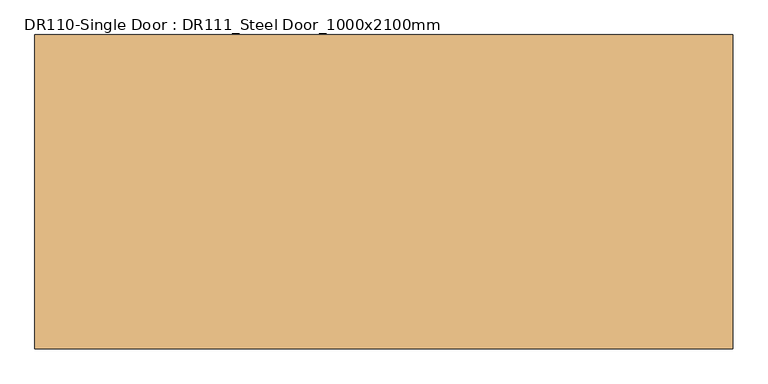
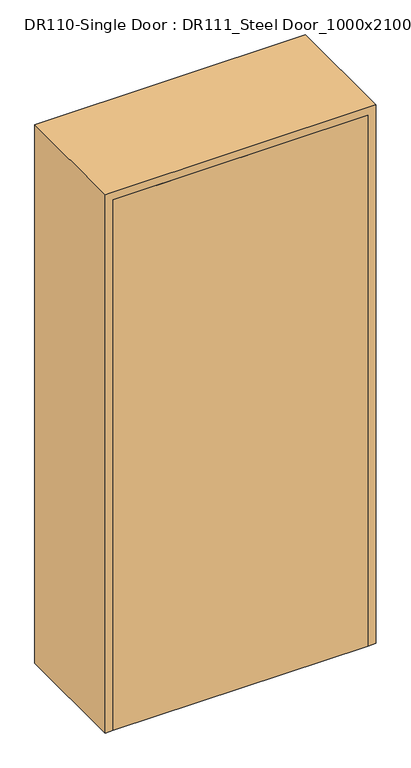
"""IFC4 building model written with IfcOpenShell, lengths in millimetres: door geometry, DR110-Single Door : DR111_Steel Door_1000x2100mm."""

from ifc_helpers import new_model, si_unit, origin, origin_with_axes, place, context, project, spatial, polyline, outline, extrude, faceted_brep, source, transform, mapped, element, save


def dr110_single_door_dr111_steel_door_1000x2100mm_3adf1b50(model_context):
    return source(origin(), model_context, "Body", "SolidModel", [
        extrude(outline(polyline([(470.0, -225.0), (-470.0, -225.0), (-470.0, -190.0), (470.0, -190.0), (470.0, -225.0)])), origin_with_axes(), (0.0, 0.0, 1.0), 2070.0),
        faceted_brep([(470.0, -225.0, 0.0), (470.0, -190.0, 0.0), (450.0, -190.0, 0.0), (450.0, 190.0, 0.0), (470.0, 190.0, 0.0), (470.0, 225.0, 0.0), (500.0, 225.0, 0.0), (500.0, -225.0, 0.0), (500.0, -225.0, 2100.0), (-500.0, -225.0, 2100.0), (-500.0, -225.0, 0.0), (-470.0, -225.0, 0.0), (-470.0, -225.0, 2070.0), (470.0, -225.0, 2070.0), (500.0, 225.0, 2100.0), (470.0, 225.0, 2070.0), (-470.0, 225.0, 2070.0), (-470.0, 225.0, 0.0), (-500.0, 225.0, 0.0), (-500.0, 225.0, 2100.0), (470.0, 190.0, 2070.0), (450.0, 190.0, 2050.0), (-450.0, 190.0, 2050.0), (-450.0, 190.0, 0.0), (-470.0, 190.0, 0.0), (-470.0, 190.0, 2070.0), (450.0, -190.0, 2050.0), (470.0, -190.0, 2070.0), (-470.0, -190.0, 2070.0), (-470.0, -190.0, 0.0), (-450.0, -190.0, 0.0), (-450.0, -190.0, 2050.0)], [[[0, 1, 2, 3, 4, 5, 6, 7]], [[7, 8, 9, 10, 11, 12, 13, 0]], [[6, 14, 8, 7]], [[5, 15, 16, 17, 18, 19, 14, 6]], [[4, 20, 15, 5]], [[3, 21, 22, 23, 24, 25, 20, 4]], [[2, 26, 21, 3]], [[1, 27, 28, 29, 30, 31, 26, 2]], [[0, 13, 27, 1]], [[12, 11, 29, 28]], [[11, 10, 18, 17, 24, 23, 30, 29]], [[19, 18, 10, 9]], [[25, 24, 17, 16]], [[31, 30, 23, 22]], [[14, 19, 9, 8]], [[20, 25, 16, 15]], [[26, 31, 22, 21]], [[13, 12, 28, 27]]]),
    ])


if __name__ == "__main__":
    model = new_model("IFC4")
    model_context = context("Model", 3, world=origin())
    ifc_project = project(units=[si_unit("LENGTHUNIT", "METRE", prefix="MILLI")], contexts=[model_context])
    site = spatial("IfcSite", under=ifc_project)
    building = spatial("IfcBuilding", under=site)
    placement = place(None, origin())
    dr110_single_door_dr111_steel_door_1000x2100mm_shape = dr110_single_door_dr111_steel_door_1000x2100mm_3adf1b50(model_context)
    element("IfcDoor", 1, ObjectType="DR110-Single Door : DR111_Steel Door_1000x2100mm", at=placement, inside=building, context=model_context, shape_type="MappedRepresentation", body=[
        mapped(dr110_single_door_dr111_steel_door_1000x2100mm_shape, transform((0.0, 0.0, 0.0), x_axis=(1.0, 0.0, 0.0), y_axis=(0.0, 1.0, 0.0), z_axis=(0.0, 0.0, 1.0))),
    ])
    save(model, "model.ifc")

# Revit data of these elements
# Type "DR110-Single Door : DR111_Steel Door_1000x2100mm"
#   Type Mark = "SD"
#   Analytic Construction = "<None>"
#   프레임 투영 외부. = 25 mm
#   프레임 투영 내부. = 25 mm
#   프레임 폭 = 75 mm
#   Height = 2100 mm
#   Width = 1000 mm
#   Define Thermal Properties by = 1
#   문 패널 = SD1 문 패널
#   문 프레임 = A04AQ098-00002_Steel Door_non FP_single
#   Function = (empty or 0)
#   Wall Closure = (empty or 0)
# Element 1 (IfcDoor, "DR110-Single Door : DR111_Steel Door_1000x2100mm")
#   Materials on its faces: "A04AQ098-00002_Steel Door_non FP_single", "SD1 문 패널"
# Materials
#   "SD1 문 패널": class "금속", colour RGB 247 247 247, transparency 0, Description = "STEEL DOOR (1000Wx2100H)"
#   "A04AQ098-00002_Steel Door_non FP_single": class "금속", colour RGB 247 247 247, transparency 0, Description = "Steel Door", W00) Work Master Code = "A04AQ098-00002", W01) Work Master_Lv1 = "Finishing Work", W02) Work Master_Lv2 = "Door & Window Work", W03) Work Master_Spec.1 = "Steel Door w/ Steel Frame", W04) Work Master_Spec.2 = "Fire Protective Rating: N/A, Single Door", W05) Work Master_Spec.3 = "w/ Hardware & Accessories", Cost = 0
